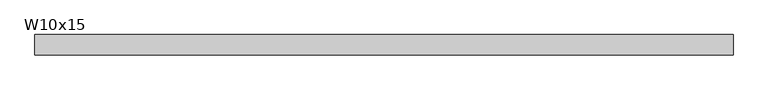
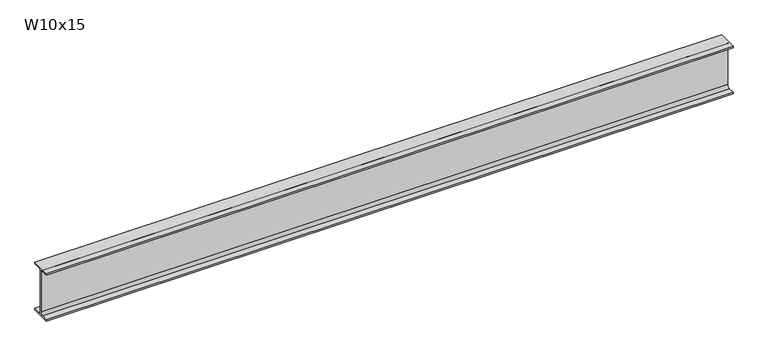
"""IFC4 building model written with IfcOpenShell, lengths in millimetres: beam geometry, RME W-Wide Flange : W10x15."""

from ifc_helpers import new_model, si_unit, point, frame, frame_2d, origin, place, context, project, spatial, polyline, circle_curve, trimmed, segment, composite_curve, outline, extrude, source, transform, mapped, element, save


def w10x15_b2536baf(model_context):
    return source(origin(), model_context, "Body", "SweptSolid", [
        extrude(outline(composite_curve([segment(polyline([(50.8, -120.142), (50.8, -127.0), (-50.8, -127.0), (-50.8, -120.142), (-16.7005, -120.142)]), True, "CONTINUOUS"), segment(trimmed(circle_curve(frame_2d((-16.7005, -106.3625)), 13.7795), [point((-16.7005, -120.142))], [point((-2.921, -106.3625))], True, "CARTESIAN"), True, "CONTINUOUS"), segment(polyline([(-2.921, -106.3625), (-2.921, 106.3625)]), True, "CONTINUOUS"), segment(trimmed(circle_curve(frame_2d((-16.7005, 106.3625)), 13.7795), [point((-2.921, 106.3625))], [point((-16.7005, 120.142))], True, "CARTESIAN"), True, "CONTINUOUS"), segment(polyline([(-16.7005, 120.142), (-50.8, 120.142), (-50.8, 127.0), (50.8, 127.0), (50.8, 120.142), (16.7005, 120.142)]), True, "CONTINUOUS"), segment(trimmed(circle_curve(frame_2d((16.7005, 106.3625)), 13.7795), [point((16.7005, 120.142))], [point((2.921, 106.3625))], True, "CARTESIAN"), True, "CONTINUOUS"), segment(polyline([(2.921, 106.3625), (2.921, -106.3625)]), True, "CONTINUOUS"), segment(trimmed(circle_curve(frame_2d((16.7005, -106.3625)), 13.7795), [point((2.921, -106.3625))], [point((16.7005, -120.142))], True, "CARTESIAN"), True, "CONTINUOUS"), segment(polyline([(16.7005, -120.142), (50.8, -120.142)]), True, "CONTINUOUS")], self_intersect=False)), frame((-1743.5077112, 0.0, 0.0), z_axis=(1.0, 0.0, 0.0), x_axis=(0.0, 1.0, 0.0)), (0.0, 0.0, 1.0), 3487.0154223),
    ])


if __name__ == "__main__":
    model = new_model("IFC4")
    model_context = context("Model", 3, world=origin())
    ifc_project = project(units=[si_unit("LENGTHUNIT", "METRE", prefix="MILLI")], contexts=[model_context])
    site = spatial("IfcSite", under=ifc_project)
    building = spatial("IfcBuilding", under=site)
    placement = place(None, origin())
    w10x15_shape = w10x15_b2536baf(model_context)
    element("IfcBeam", 1, ObjectType="RME W-Wide Flange : W10x15", at=placement, inside=building, context=model_context, shape_type="MappedRepresentation", body=[
        mapped(w10x15_shape, transform((0.0, 0.0, 0.0), x_axis=(1.0, 0.0, 0.0), y_axis=(0.0, 1.0, 0.0), z_axis=(0.0, 0.0, 1.0))),
    ])
    save(model, "model.ifc")

# Revit data of these elements
# Type "RME W-Wide Flange : W10x15"
#   WELD P [instance default] = ""
#   WELD LE [instance default] = ""
#   WELD D [instance default] = ""
#   TOP SECTION SIZE [instance default] = ""
#   TOP SECTION LENGTH [instance default] = ""
#   REMARKS [instance default] = ""
#   REINF TYPE [instance default] = ""
#   Nominal Size = "W24"
#   End Bearing Capacity [instance default] = ""
#   BOT SECTION SIZE [instance default] = ""
#   BOT SECTION LENGTH [instance default] = ""
#   Assembly Code = "B10"
#   W = 15
#   Start Extension Calculation [instance default] = 10' - 0"
#   Start Extension [instance default] = -0' - 0 1/2"
#   End Extension Calculation [instance default] = 10' - 0"
#   End Extension [instance default] = -0' - 0 1/2"
#   Length [instance default] = 5' - 0"
#   bf = 0' - 4"
#   d = 0' - 10"
#   k = 0' - 0 13/16"
#   k2 = 0' - 0.5425"
#   tf = 0' - 0.27"
#   tw = 0' - 0.23"
#   A = 0.030625 SF
#   Structural Material [instance default] = Metal - Steel - ASTM A992
# Element 1 (IfcBeam, "RME W-Wide Flange : W10x15")
#   Length = 11' - 5.28407"
#   Materials on its faces: "Metal - Steel - ASTM A992"
# Materials
#   "Metal - Steel - ASTM A992": class "Metal", colour RGB 255 128 0, transparency 0
